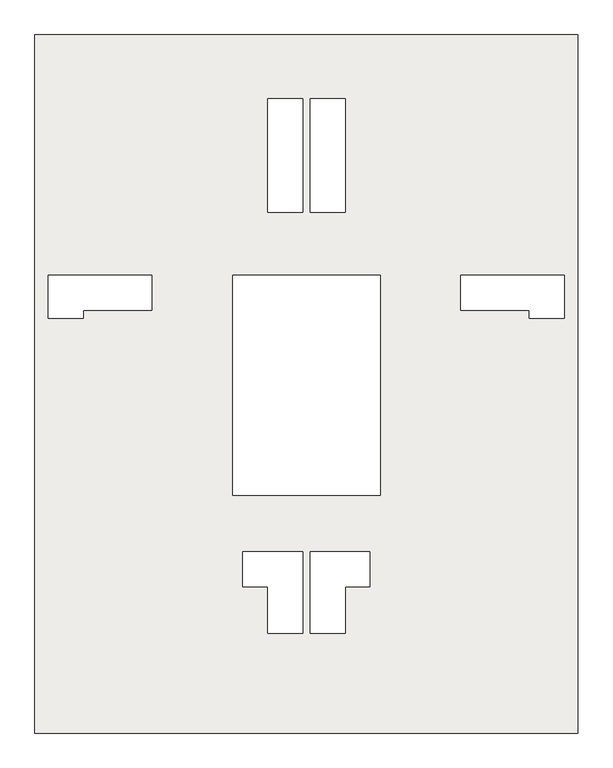
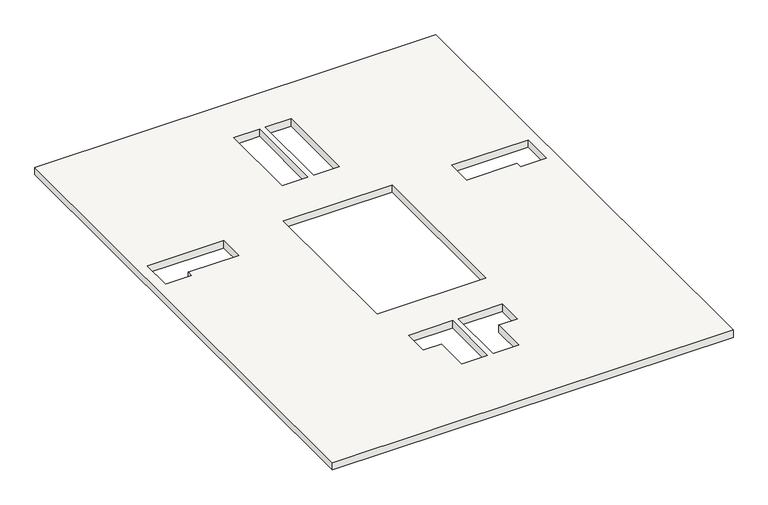
"""IFC4 building model written with IfcOpenShell, lengths in millimetres: slab geometry, Holzdecke."""

from ifc_helpers import new_model, si_unit, origin, origin_with_axes, place, context, project, spatial, polyline, outline, extrude, source, transform, mapped, element, save


def slab_c00a345a(model_context):
    return source(origin(), model_context, "Body", "SweptSolid", [
        extrude(outline(polyline([(14000.0, 0.0), (0.0, 0.0), (0.0, 18002.8619019), (14000.0, 18002.8619019), (14000.0, 0.0)]), holes=[polyline([(3014.6018366, 10902.8619019), (3014.6018366, 11802.8619019), (350.0, 11802.8619019), (350.0, 10698.126196), (1250.0, 10698.126196), (1250.0, 10902.8619019), (3014.6018366, 10902.8619019)]), polyline([(7100.0, 4677.8619019), (7100.0, 2573.2600653), (8000.0, 2573.2600653), (8000.0, 3777.8619019), (8640.0, 3777.8619019), (8640.0, 4677.8619019), (7100.0, 4677.8619019)]), polyline([(5360.0, 3777.8619019), (6000.0, 3777.8619019), (6000.0, 2573.2600653), (6900.0, 2573.2600653), (6900.0, 4677.8619019), (5360.0, 4677.8619019), (5360.0, 3777.8619019)]), polyline([(12750.0, 10902.8619019), (12750.0, 10698.126196), (13650.0, 10698.126196), (13650.0, 11802.8619019), (10985.3981634, 11802.8619019), (10985.3981634, 10902.8619019), (12750.0, 10902.8619019)]), polyline([(8000.0, 16360.6619019), (7100.0, 16360.6619019), (7100.0, 13432.8619019), (8000.0, 13432.8619019), (8000.0, 16360.6619019)]), polyline([(6000.0, 13432.8619019), (6900.0, 13432.8619019), (6900.0, 16360.6619019), (6000.0, 16360.6619019), (6000.0, 13432.8619019)]), polyline([(5100.0, 11802.8619019), (5100.0, 6132.8619019), (8900.0, 6132.8619019), (8900.0, 11802.8619019), (5100.0, 11802.8619019)])]), origin_with_axes(), (0.0, 0.0, 1.0), 270.0),
    ])


if __name__ == "__main__":
    model = new_model("IFC4")
    model_context = context("Model", 3, world=origin())
    ifc_project = project(units=[si_unit("LENGTHUNIT", "METRE", prefix="MILLI")], contexts=[model_context])
    site = spatial("IfcSite", under=ifc_project)
    building = spatial("IfcBuilding", under=site)
    placement = place(None, origin())
    slab_shape = slab_c00a345a(model_context)
    element("IfcSlab", 1, ObjectType="Holzdecke", at=placement, inside=building, context=model_context, shape_type="MappedRepresentation", body=[
        mapped(slab_shape, transform((0.0, 0.0, 0.0), x_axis=(1.0, 0.0, 0.0), y_axis=(0.0, 1.0, 0.0), z_axis=(0.0, 0.0, 1.0))),
    ])
    save(model, "model.ifc")

# Revit data of these elements
# Element 1 (IfcSlab, "Holzdecke")
#   Materials on its faces: "holzschalung"
# Materials
#   "holzschalung": class "Unassigned", colour RGB 128 128 128, transparency 0
